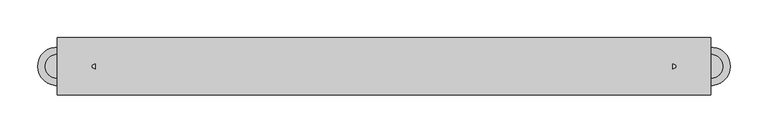
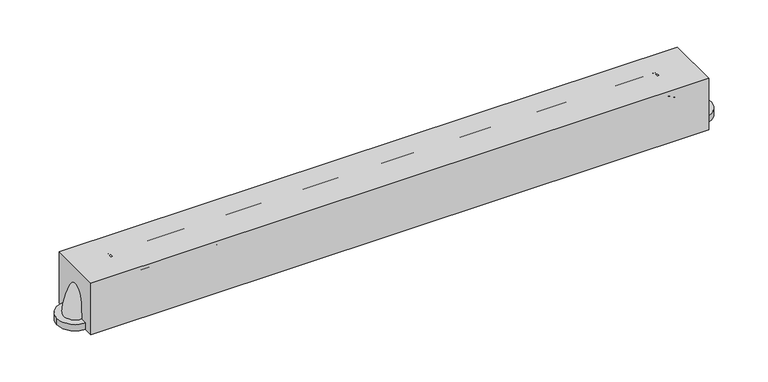
"""IFC4 building model written with IfcOpenShell, lengths in millimetres: proxy geometry, A5109 - Grab Bar, 1.25 in Dia, SS, 2 Wall, W-C Accessible : A5109 - Grab Bar, 1.25 in Dia, SS, 2 Wall, W-C Accessible."""

from ifc_helpers import new_model, si_unit, point, frame, frame_2d, origin, origin_with_axes, place, context, project, spatial, polyline, circle_curve, ellipse_curve, trimmed, segment, composite_curve, outline, extrude, source, transform, mapped, element, save
from ifc_brep_helpers import plane_surface, revolved_surface, advanced_brep


def specialty_equipment_717dfb8c(model_context):
    return source(origin(), model_context, "Body", "SolidModel", [
        advanced_brep(
        [(381.7182679, 15.875, 60.325), (381.7182679, -15.875, 60.325), (432.5182679, 15.875, 9.525), (432.5182679, -15.875, 9.525)],
        [
            (0, 1, circle_curve(frame((381.7182679, 0.0, 60.325), z_axis=(-1.0, 0.0, 0.0), x_axis=(0.0, -1.0, 0.0)), 15.875)),
            (1, 0, circle_curve(frame((381.7182679, 0.0, 60.325), z_axis=(-1.0, 0.0, 0.0), x_axis=(0.0, -1.0, 0.0)), 15.875)),
            (2, 3, circle_curve(frame((432.5182679, 0.0, 9.525), z_axis=(0.0, 0.0, -1.0), x_axis=(0.0, -1.0, 0.0)), 15.875)),
            (3, 2, circle_curve(frame((432.5182679, 0.0, 9.525), z_axis=(0.0, 0.0, -1.0), x_axis=(0.0, -1.0, 0.0)), 15.875)),
            (2, 0, circle_curve(frame((381.7182679, 15.875, 9.525), z_axis=(0.0, -1.0, 0.0), x_axis=(0.0, 0.0, 1.0)), 50.8)),
            (1, 3, circle_curve(frame((381.7182679, -15.875, 9.525), z_axis=(0.0, 1.0, 0.0), x_axis=(0.0, 0.0, 1.0)), 50.8)),
        ],
        [
            plane_surface(frame((381.7182679, 0.0, 60.325), z_axis=(-1.0, 0.0, 0.0), x_axis=(0.0, -1.0, 0.0))),
            plane_surface(frame((432.5182679, 0.0, 9.525), z_axis=(0.0, 0.0, -1.0), x_axis=(0.0, -1.0, 0.0))),
            revolved_surface(trimmed(ellipse_curve(frame((381.7182679, 0.0, 60.325), z_axis=(1.0, 0.0, 0.0), x_axis=(0.0, -1.0, 0.0)), 15.875, 15.875), [point((381.7182679, 15.875, 60.325))], [point((381.7182679, -15.875, 60.325))], True, "CARTESIAN"), (381.7182679, 0.0, 9.525), (0.0, -1.0, 0.0)),
            revolved_surface(trimmed(ellipse_curve(frame((381.7182679, 0.0, 60.325), z_axis=(1.0, 0.0, 0.0), x_axis=(0.0, -1.0, 0.0)), 15.875, 15.875), [point((381.7182679, -15.875, 60.325))], [point((381.7182679, 15.875, 60.325))], True, "CARTESIAN"), (381.7182679, 0.0, 9.525), (0.0, -1.0, 0.0)),
        ],
        [
            (0, [[1, 2]]),
            (1, [[3, 4]]),
            (2, [[-3, 5, -2, 6]]),
            (3, [[-4, -6, -1, -5]]),
        ],
    ),
        extrude(outline(composite_curve([segment(trimmed(circle_curve(frame_2d((432.5182679, 0.0)), 25.4), [point((457.9182679, 0.0))], [point((407.1182679, 0.0))], False, "CARTESIAN"), True, "CONTINUOUS"), segment(trimmed(circle_curve(frame_2d((432.5182679, 0.0)), 25.4), [point((407.1182679, 0.0))], [point((457.9182679, 0.0))], False, "CARTESIAN"), True, "CONTINUOUS")], self_intersect=False)), origin_with_axes(), (0.0, 0.0, 1.0), 9.525),
        advanced_brep(
        [(-381.7182679, 15.875, 60.325), (-381.7182679, -15.875, 60.325), (-432.5182679, 15.875, 9.525), (-432.5182679, -15.875, 9.525)],
        [
            (0, 1, circle_curve(frame((-381.7182679, 0.0, 60.325), z_axis=(1.0, 0.0, 0.0), x_axis=(0.0, -1.0, 0.0)), 15.875)),
            (1, 0, circle_curve(frame((-381.7182679, 0.0, 60.325), z_axis=(1.0, 0.0, 0.0), x_axis=(0.0, -1.0, 0.0)), 15.875)),
            (2, 3, circle_curve(frame((-432.5182679, 0.0, 9.525), z_axis=(0.0, 0.0, -1.0), x_axis=(0.0, -1.0, 0.0)), 15.875)),
            (3, 2, circle_curve(frame((-432.5182679, 0.0, 9.525), z_axis=(0.0, 0.0, -1.0), x_axis=(0.0, -1.0, 0.0)), 15.875)),
            (3, 1, circle_curve(frame((-381.7182679, -15.875, 9.525), z_axis=(0.0, 1.0, 0.0), x_axis=(0.0, 0.0, 1.0)), 50.8)),
            (0, 2, circle_curve(frame((-381.7182679, 15.875, 9.525), z_axis=(0.0, -1.0, 0.0), x_axis=(0.0, 0.0, 1.0)), 50.8)),
        ],
        [
            plane_surface(frame((-381.7182679, 0.0, 60.325), z_axis=(1.0, 0.0, 0.0), x_axis=(0.0, -1.0, 0.0))),
            plane_surface(frame((-432.5182679, 0.0, 9.525), z_axis=(0.0, 0.0, -1.0), x_axis=(0.0, -1.0, 0.0))),
            revolved_surface(trimmed(ellipse_curve(frame((-381.7182679, 0.0, 60.325), z_axis=(1.0, 0.0, 0.0), x_axis=(0.0, -1.0, 0.0)), 15.875, 15.875), [point((-381.7182679, 15.875, 60.325))], [point((-381.7182679, -15.875, 60.325))], True, "CARTESIAN"), (-381.7182679, 0.0, 9.525), (0.0, -1.0, 0.0)),
            revolved_surface(trimmed(ellipse_curve(frame((-381.7182679, 0.0, 60.325), z_axis=(1.0, 0.0, 0.0), x_axis=(0.0, -1.0, 0.0)), 15.875, 15.875), [point((-381.7182679, -15.875, 60.325))], [point((-381.7182679, 15.875, 60.325))], True, "CARTESIAN"), (-381.7182679, 0.0, 9.525), (0.0, -1.0, 0.0)),
        ],
        [
            (0, [[1, 2]]),
            (1, [[3, 4]]),
            (2, [[5, -1, 6, -4]]),
            (3, [[-6, -2, -5, -3]]),
        ],
    ),
        extrude(outline(composite_curve([segment(trimmed(circle_curve(frame_2d((-432.5182679, 0.0)), 25.4), [point((-457.9182679, 0.0))], [point((-407.1182679, 0.0))], False, "CARTESIAN"), True, "CONTINUOUS"), segment(trimmed(circle_curve(frame_2d((-432.5182679, 0.0)), 25.4), [point((-407.1182679, 0.0))], [point((-457.9182679, 0.0))], False, "CARTESIAN"), True, "CONTINUOUS")], self_intersect=False)), origin_with_axes(), (0.0, 0.0, 1.0), 9.525),
        extrude(outline(polyline([(432.5182679, -38.1), (-432.5182679, -38.1), (-432.5182679, 38.1), (432.5182679, 38.1), (432.5182679, -38.1)])), origin_with_axes(), (0.0, 0.0, 1.0), 76.2),
        extrude(outline(composite_curve([segment(trimmed(circle_curve(frame_2d((0.0, 60.325)), 15.875), [point((-15.875, 60.325))], [point((15.875, 60.325))], False, "CARTESIAN"), True, "CONTINUOUS"), segment(trimmed(circle_curve(frame_2d((0.0, 60.325)), 15.875), [point((15.875, 60.325))], [point((-15.875, 60.325))], False, "CARTESIAN"), True, "CONTINUOUS")], self_intersect=False)), frame((-381.7182679, 0.0, 0.0), z_axis=(1.0, 0.0, 0.0), x_axis=(0.0, 1.0, 0.0)), (0.0, 0.0, 1.0), 763.4365358),
    ])


if __name__ == "__main__":
    model = new_model("IFC4")
    model_context = context("Model", 3, world=origin())
    ifc_project = project(units=[si_unit("LENGTHUNIT", "METRE", prefix="MILLI")], contexts=[model_context])
    site = spatial("IfcSite", under=ifc_project)
    building = spatial("IfcBuilding", under=site)
    placement = place(None, origin())
    specialty_equipment_shape = specialty_equipment_717dfb8c(model_context)
    element("IfcBuildingElementProxy", 1, Name="A5109 - Grab Bar, 1.25 in Dia, SS, 2 Wall, W-C Accessible : A5109 - Grab Bar, 1.25 in Dia, SS, 2 Wall, W-C Accessible", ObjectType="A5109 - Grab Bar, 1.25 in Dia, SS, 2 Wall, W-C Accessible : A5109 - Grab Bar, 1.25 in Dia, SS, 2 Wall, W-C Accessible", at=placement, inside=building, context=model_context, shape_type="MappedRepresentation", body=[
        mapped(specialty_equipment_shape, transform((0.0, 0.0, 0.0), x_axis=(1.0, 0.0, 0.0), y_axis=(0.0, 1.0, 0.0), z_axis=(0.0, 0.0, 1.0))),
    ])
    save(model, "model.ifc")

# Revit data of these elements
# Type "A5109 - Grab Bar, 1.25 in Dia, SS, 2 Wall, W-C Accessible : A5109 - Grab Bar, 1.25 in Dia, SS, 2 Wall, W-C Accessible"
#   Watts2 = "0"
#   Watts1 = "0"
#   Unit_Issue = "EA"
#   UTIL_6_Misc = "-"
#   UTIL_5_NonMedGas = "-"
#   UTIL_4_MiscGas = "-"
#   UTIL_3_MedGas = "-"
#   UTIL_2_Elec = "-"
#   UTIL_1_WaterDrain = "-"
#   Nomenclature = "Grab Bar, 1-1/4\" Dia., SS, 2 Wall, W/C Accessible"
#   NSN = "6530"
#   Location [instance default] = ""
#   JSN = "A5109"
#   Fund_Source_VA = "-"
#   Fund_Source_Navy = "-"
#   Fund_Source_Army = "-"
#   Fund_Source_AF = "-"
#   ELEC_Volts2 = "0"
#   ELEC_Volts1 = "0"
#   ELEC_Phase2 = "0"
#   ELEC_Phase1 = "0"
#   ELEC_HertzSwitch = "0"
#   ELEC_HertzDependent = "0"
#   ELEC_Hertz = "0"
#   ELEC_Amps2 = "0"
#   ELEC_Amps1 = "0"
#   DetailDescription = "A 1-1/4\" diameter, satin finish stainless steel, peened gripping surface, 2 wall toilet stall/ room, grab bar with concealed mounting flanges.  Snap over flanges are provided to conceal mounting screws. A selection of mounting kits and concealed anchor devices are available from the manufacturers for different types of installations. Grab bar shall comply with barrier-free accessibility guidelines for structural strength. For typical water closet applications in toilet stalls and rooms where ADA (American''s With Disabilities Act) requirements must be met."
#   CAT_VA = "A"
#   CAT_Navy = "A"
#   CAT_IHS = "-"
#   CAT_Army = "A"
#   CAT_AF = "A"
#   BTUperhour = "0"
#   Weight_IP = 7
#   Default Elevation = 2' - 9"
#   DIM_Width_IP = 4' - 9"
#   DIM_Height_IP = 0' - 3"
#   DIM_Depth_IP = 0' - 3"
#   CustomLength [instance default] = 2' - 0"
# Element 1 (IfcBuildingElementProxy, "A5109 - Grab Bar, 1.25 in Dia, SS, 2 Wall, W-C Accessible : A5109 - Grab Bar, 1.25 in Dia, SS, 2 Wall, W-C Accessible")
#   Location = "TLTS1"
#   CustomLength = 2' - 10.05656"
#   Materials on its faces: "EquipSpace"
# Materials
#   "EquipSpace": class "Unassigned", colour RGB 221 217 195, transparency 0.5
